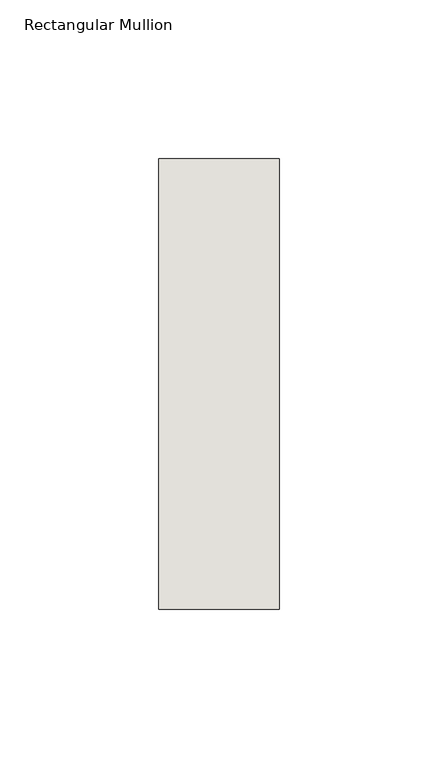
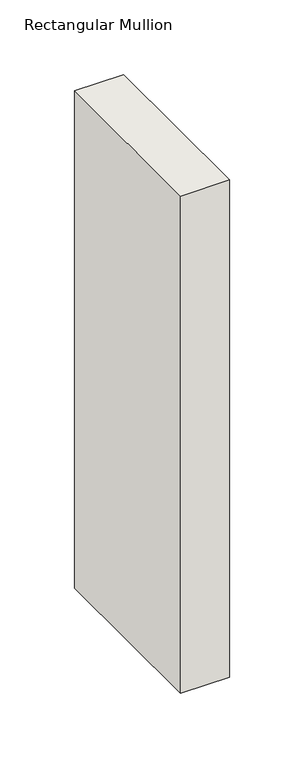
"""IFC4 building model written with IfcOpenShell, lengths in millimetres: wall geometry, Rectangular Mullion : NLRS_21_CWM_hsb-regel 38x142_gen_rsf."""

from ifc_helpers import new_model, si_unit, frame, origin, place, context, project, spatial, polyline, outline, extrude, source, transform, mapped, element, save


def rectangular_mullion_b195b317(model_context):
    return source(origin(), model_context, "Body", "SweptSolid", [
        extrude(outline(polyline([(-38.0, -71.0), (-38.0, 71.0), (0.0, 71.0), (0.0, -71.0), (-38.0, -71.0)])), frame((0.0, 0.0, -407.0000003), z_axis=(0.0, 0.0, 1.0), x_axis=(1.0, 0.0, 0.0)), (0.0, 0.0, 1.0), 407.0000003),
    ])


if __name__ == "__main__":
    model = new_model("IFC4")
    model_context = context("Model", 3, world=origin())
    ifc_project = project(units=[si_unit("LENGTHUNIT", "METRE", prefix="MILLI")], contexts=[model_context])
    site = spatial("IfcSite", under=ifc_project)
    building = spatial("IfcBuilding", under=site)
    placement = place(None, origin())
    rectangular_mullion_shape = rectangular_mullion_b195b317(model_context)
    element("IfcWall", 1, ObjectType="Rectangular Mullion : NLRS_21_CWM_hsb-regel 38x142_gen_rsf", at=placement, inside=building, context=model_context, shape_type="MappedRepresentation", body=[
        mapped(rectangular_mullion_shape, transform((0.0, 0.0, 0.0), x_axis=(1.0, 0.0, 0.0), y_axis=(0.0, 1.0, 0.0), z_axis=(0.0, 0.0, 1.0))),
    ])
    save(model, "model.ifc")

# Revit data of these elements
# Type "Rectangular Mullion : NLRS_21_CWM_hsb-regel 38x142_gen_rsf"
#   Type IfcGUID = "07M7mRoiH1CR8m_RSKIwpF"
#   Assembly Code = "21.10"
#   IfcExportAs = "IfcWall"
#   built-in parameter 1007322 = 0.465879 (stored number, unit not read)
#   built-in parameter 1007321 = 0.062336 (stored number, unit not read)
#   built-in parameter 1007320 = 0.062336 (stored number, unit not read)
# Element 1 (IfcWall, "Rectangular Mullion : NLRS_21_CWM_hsb-regel 38x142_gen_rsf")
#   Materials on its faces: "NLRS_i2_hout naaldhout vuren_gen_rsf"
# Materials
#   "NLRS_i2_hout naaldhout vuren_gen_rsf": class "I - Hout", colour RGB 234 199 147, transparency 0, Keynote = "i2", Manufacturer = "Revit Standards Foundation", URL = "www.revitstandards.org", Description = "hout vuren", Cost = 0
